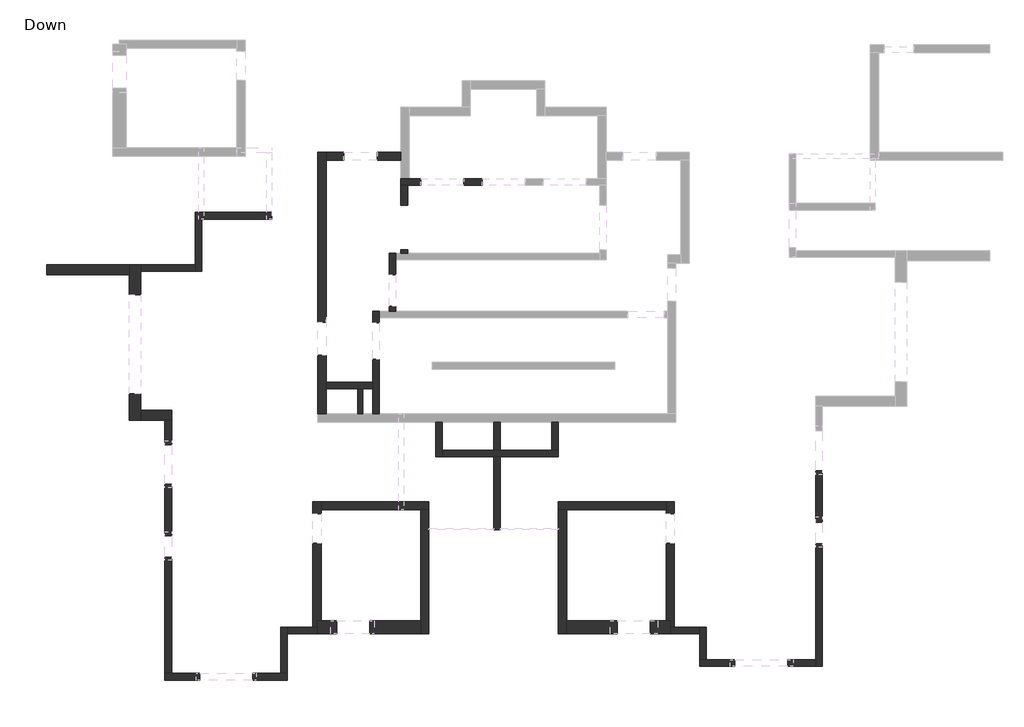
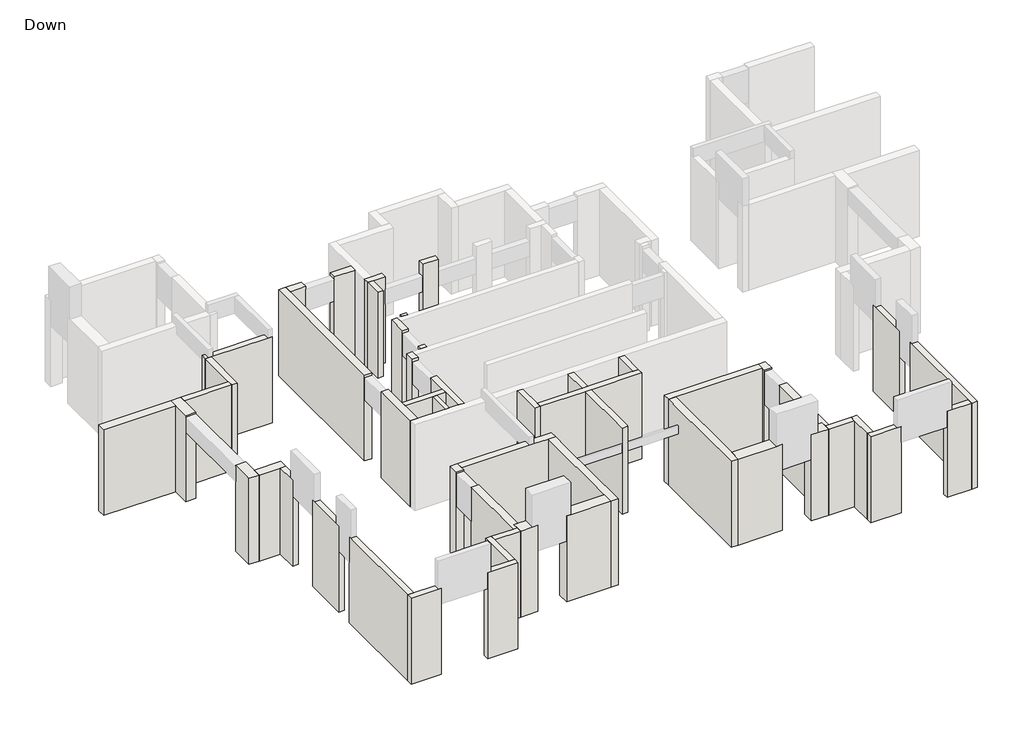
# One storey, part 1 of 3: 51 walls.
# Revit data of these elements (continued)
# Element 19 (IfcWall, "20") (continued)
#   Base Constraint = Down
#   Top Constraint = Typical Floor
#   Materials on its faces: "Concrete"
# Element 20 (IfcWall, "20")
#   Comments = ""
#   Mark = "W54"
#   SOFiSTiK_EdgeZones = "W54"
#   SOFiSTiK_AMG_Comments = ""
#   Top Offset = 0 cm
#   Base Offset = 0 cm
#   wall height = 315 cm
#   SOFiSTiK_AMG_Scheduled = yes
#   SOFiSTiK_AMG_Adjusted = yes
#   Phase Created = New Construction
#   Base Constraint = Down
#   Top Constraint = Typical Floor
#   Materials on its faces: "Concrete"
# Element 21 (IfcWall, "20")
#   Comments = ""
#   Mark = "W55"
#   SOFiSTiK_EdgeZones = "W55"
#   SOFiSTiK_AMG_Comments = ""
#   Top Offset = 0 cm
#   Base Offset = 0 cm
#   wall height = 315 cm
#   SOFiSTiK_AMG_Scheduled = yes
#   SOFiSTiK_AMG_Adjusted = yes
#   Phase Created = New Construction
#   Base Constraint = Down
#   Top Constraint = Typical Floor
#   Materials on its faces: "Concrete"
# Element 22 (IfcWall, "20")
#   Comments = ""
#   Mark = "W56"
#   SOFiSTiK_EdgeZones = "W56"
#   SOFiSTiK_AMG_Comments = ""
#   Top Offset = 0 cm
#   Base Offset = 0 cm
#   wall height = 315 cm
#   SOFiSTiK_AMG_Scheduled = yes
#   SOFiSTiK_AMG_Adjusted = yes
#   Phase Created = New Construction
#   Base Constraint = Down
#   Top Constraint = Typical Floor
#   Materials on its faces: "Concrete"
# Element 23 (IfcWall, "20")
#   Comments = ""
#   Mark = "W57"
#   SOFiSTiK_EdgeZones = "W57"
#   SOFiSTiK_AMG_Comments = ""
#   Top Offset = 0 cm
#   Base Offset = 0 cm
#   wall height = 315 cm
#   SOFiSTiK_AMG_Scheduled = yes
#   SOFiSTiK_AMG_Adjusted = yes
#   Phase Created = New Construction
#   Base Constraint = Down
#   Top Constraint = Typical Floor
#   Materials on its faces: "Concrete"
# Element 24 (IfcWall, "20")
#   Comments = ""
#   Mark = "W58"
#   SOFiSTiK_EdgeZones = "W58"
#   SOFiSTiK_AMG_Comments = ""
#   Top Offset = 0 cm
#   Base Offset = 0 cm
#   wall height = 315 cm
#   SOFiSTiK_AMG_Scheduled = yes
#   SOFiSTiK_AMG_Adjusted = yes
#   Phase Created = New Construction
#   Base Constraint = Down
#   Top Constraint = Typical Floor
#   Materials on its faces: "Concrete"
# Element 25 (IfcWall, "20")
#   Comments = ""
#   Mark = "W59"
#   SOFiSTiK_EdgeZones = "W59"
#   SOFiSTiK_AMG_Comments = ""
#   Top Offset = 0 cm
#   Base Offset = 0 cm
#   wall height = 315 cm
#   SOFiSTiK_AMG_Scheduled = yes
#   SOFiSTiK_AMG_Adjusted = yes
#   Phase Created = New Construction
#   Base Constraint = Down
#   Top Constraint = Typical Floor
#   Materials on its faces: "Concrete"
# Element 26 (IfcWall, "20")
#   Comments = ""
#   Mark = "W60"
#   SOFiSTiK_EdgeZones = "W60"
#   SOFiSTiK_AMG_Comments = ""
#   Top Offset = 0 cm
#   Base Offset = 0 cm
#   wall height = 315 cm
#   SOFiSTiK_AMG_Scheduled = yes
#   SOFiSTiK_AMG_Adjusted = yes
#   Phase Created = New Construction
#   Base Constraint = Down
#   Top Constraint = Typical Floor
#   Materials on its faces: "Concrete"
# Element 27 (IfcWall, "20")
#   Comments = ""
#   Mark = "W61"
#   SOFiSTiK_EdgeZones = "W61"
#   SOFiSTiK_AMG_Comments = ""
#   Top Offset = 0 cm
#   Base Offset = 0 cm
#   wall height = 315 cm
#   SOFiSTiK_AMG_Scheduled = yes
#   SOFiSTiK_AMG_Adjusted = yes
#   Phase Created = New Construction
#   Base Constraint = Down
#   Top Constraint = Typical Floor
#   Materials on its faces: "Concrete"
# Element 28 (IfcWall, "20")
#   Comments = ""
#   Mark = "W69"
#   SOFiSTiK_EdgeZones = "W69"
#   SOFiSTiK_AMG_Comments = ""
#   Top Offset = 0 cm
#   Base Offset = 0 cm
#   wall height = 315 cm
#   SOFiSTiK_AMG_Scheduled = yes
#   SOFiSTiK_AMG_Adjusted = yes
#   Phase Created = New Construction
#   Base Constraint = Down
#   Top Constraint = Typical Floor
#   Materials on its faces: "Concrete"
# Element 29 (IfcWall, "20")
#   Comments = ""
#   Mark = "W71"
#   SOFiSTiK_EdgeZones = "W71"
#   SOFiSTiK_AMG_Comments = ""
#   Top Offset = 0 cm
#   Base Offset = 0 cm
#   wall height = 315 cm
#   SOFiSTiK_AMG_Scheduled = yes
#   SOFiSTiK_AMG_Adjusted = yes
#   Phase Created = New Construction
#   Base Constraint = Down
#   Top Constraint = Typical Floor
#   Materials on its faces: "Concrete"
# Element 30 (IfcWall, "20")
#   Comments = ""
#   Mark = "W72"
#   SOFiSTiK_EdgeZones = "W72"
#   SOFiSTiK_AMG_Comments = ""
#   Top Offset = 0 cm
#   Base Offset = 0 cm
#   wall height = 315 cm
#   SOFiSTiK_AMG_Scheduled = yes
#   SOFiSTiK_AMG_Adjusted = yes
#   Phase Created = New Construction
#   Base Constraint = Down
#   Top Constraint = Typical Floor
#   Materials on its faces: "Concrete"
# Element 31 (IfcWall, "20")
#   Comments = ""
#   Mark = "W73"
#   SOFiSTiK_EdgeZones = "W73"
#   SOFiSTiK_AMG_Comments = ""
#   Top Offset = 0 cm
#   Base Offset = 0 cm
#   wall height = 315 cm
#   SOFiSTiK_AMG_Scheduled = yes
#   SOFiSTiK_AMG_Adjusted = yes
#   Phase Created = New Construction
#   Base Constraint = Down
#   Top Constraint = Typical Floor
#   Materials on its faces: "Concrete"
# Element 32 (IfcWall, "25")
#   Comments = ""
#   Mark = "W90"
#   SOFiSTiK_EdgeZones = "W90"
#   SOFiSTiK_AMG_Comments = ""
#   Top Offset = 0 cm
#   Base Offset = 0 cm
#   wall height = 315 cm
#   SOFiSTiK_AMG_Scheduled = yes
#   SOFiSTiK_AMG_Adjusted = yes
#   Phase Created = New Construction
#   Base Constraint = Down
#   Top Constraint = Typical Floor
#   Materials on its faces: "Concrete"
# Element 33 (IfcWall, "25")
#   Comments = ""
#   Mark = "W91"
#   SOFiSTiK_EdgeZones = "W91"
#   SOFiSTiK_AMG_Comments = ""
#   Top Offset = 0 cm
#   Base Offset = 0 cm
#   wall height = 315 cm
#   SOFiSTiK_AMG_Scheduled = yes
#   SOFiSTiK_AMG_Adjusted = yes
#   Phase Created = New Construction
#   Base Constraint = Down
#   Top Constraint = Typical Floor
#   Materials on its faces: "Concrete"
# Element 34 (IfcWall, "25")
#   Comments = ""
#   Mark = "W92"
#   SOFiSTiK_EdgeZones = "W92"
#   SOFiSTiK_AMG_Comments = ""
#   Top Offset = 0 cm
#   Base Offset = 0 cm
#   wall height = 315 cm
#   SOFiSTiK_AMG_Scheduled = yes
#   SOFiSTiK_AMG_Adjusted = yes
#   Phase Created = New Construction
#   Base Constraint = Down
#   Top Constraint = Typical Floor
#   Materials on its faces: "Concrete"
# Element 35 (IfcWall, "25")
#   Comments = ""
#   Mark = "W93"
#   SOFiSTiK_EdgeZones = "W93"
#   SOFiSTiK_AMG_Comments = ""
#   Top Offset = 0 cm
#   Base Offset = 0 cm
#   wall height = 315 cm
#   SOFiSTiK_AMG_Scheduled = yes
#   SOFiSTiK_AMG_Adjusted = yes
#   Phase Created = New Construction
#   Base Constraint = Down
#   Top Constraint = Typical Floor
#   Materials on its faces: "Concrete"
# Element 36 (IfcWall, "25")
#   Comments = ""
#   Mark = "W94"
#   SOFiSTiK_EdgeZones = "W94"
#   SOFiSTiK_AMG_Comments = ""
#   Top Offset = 0 cm
#   Base Offset = 0 cm
#   wall height = 315 cm
#   SOFiSTiK_AMG_Scheduled = yes
#   SOFiSTiK_AMG_Adjusted = yes
#   Phase Created = New Construction
#   Base Constraint = Down
#   Top Constraint = Typical Floor
#   Materials on its faces: "Concrete"
# Element 37 (IfcWall, "25")
#   Comments = ""
#   Mark = "W95"
#   SOFiSTiK_EdgeZones = "W95"
#   SOFiSTiK_AMG_Comments = ""
#   Top Offset = 0 cm
#   Base Offset = 0 cm
#   wall height = 315 cm
#   SOFiSTiK_AMG_Scheduled = yes
#   SOFiSTiK_AMG_Adjusted = yes
#   Phase Created = New Construction
#   Base Constraint = Down
#   Top Constraint = Typical Floor
#   Materials on its faces: "Concrete"
# Element 38 (IfcWall, "25")
#   Comments = ""
#   Mark = "W96"
#   SOFiSTiK_EdgeZones = "W96"
#   SOFiSTiK_AMG_Comments = ""
#   Top Offset = 0 cm
#   Base Offset = 0 cm
#   wall height = 315 cm
#   SOFiSTiK_AMG_Scheduled = yes
#   SOFiSTiK_AMG_Adjusted = yes
#   Phase Created = New Construction
#   Base Constraint = Down
#   Top Constraint = Typical Floor
#   Materials on its faces: "Concrete"
# Element 39 (IfcWall, "25")
#   Comments = ""
#   Mark = "W97"
#   SOFiSTiK_EdgeZones = "W97"
#   SOFiSTiK_AMG_Comments = ""
#   Top Offset = 0 cm
#   Base Offset = 0 cm
#   wall height = 315 cm
#   SOFiSTiK_AMG_Scheduled = yes
#   SOFiSTiK_AMG_Adjusted = yes
#   Phase Created = New Construction
#   Base Constraint = Down
#   Top Constraint = Typical Floor
#   Materials on its faces: "Concrete"
# Element 40 (IfcWall, "25")
#   Comments = ""
#   Mark = "W100"
#   SOFiSTiK_EdgeZones = "W100"
#   SOFiSTiK_AMG_Comments = ""
#   Top Offset = 0 cm
#   Base Offset = 0 cm
#   wall height = 315 cm
#   SOFiSTiK_AMG_Scheduled = yes
#   SOFiSTiK_AMG_Adjusted = yes
#   Phase Created = New Construction
#   Base Constraint = Down
#   Top Constraint = Typical Floor
#   Materials on its faces: "Concrete"
# Element 41 (IfcWall, "25")
#   Comments = ""
#   Mark = "W101"
#   SOFiSTiK_EdgeZones = "W101"
#   SOFiSTiK_AMG_Comments = ""
#   Top Offset = 0 cm
#   Base Offset = 0 cm
#   wall height = 315 cm
#   SOFiSTiK_AMG_Scheduled = yes
#   SOFiSTiK_AMG_Adjusted = yes
#   Phase Created = New Construction
#   Base Constraint = Down
#   Top Constraint = Typical Floor
#   Materials on its faces: "Concrete"
# Element 42 (IfcWall, "25")
#   Comments = ""
#   Mark = "W102"
#   SOFiSTiK_EdgeZones = "W102"
#   SOFiSTiK_AMG_Comments = ""
#   Top Offset = 0 cm
#   Base Offset = 0 cm
#   wall height = 315 cm
#   SOFiSTiK_AMG_Scheduled = yes
#   SOFiSTiK_AMG_Adjusted = yes
#   Phase Created = New Construction
#   Base Constraint = Down
#   Top Constraint = Typical Floor
#   Materials on its faces: "Concrete"
# Element 43 (IfcWall, "25")
#   Comments = ""
#   Mark = "W103"
#   SOFiSTiK_EdgeZones = "W103"
#   SOFiSTiK_AMG_Comments = ""
#   Top Offset = 0 cm
#   Base Offset = 0 cm
#   wall height = 315 cm
#   SOFiSTiK_AMG_Scheduled = yes
#   SOFiSTiK_AMG_Adjusted = yes
#   Phase Created = New Construction
#   Base Constraint = Down
#   Top Constraint = Typical Floor
#   Materials on its faces: "Concrete"
# Element 44 (IfcWall, "30")
#   Comments = ""
#   Mark = "W77"
#   SOFiSTiK_EdgeZones = "W77"
#   SOFiSTiK_AMG_Comments = ""
#   Top Offset = 0 cm
#   Base Offset = 0 cm
#   wall height = 315 cm
#   SOFiSTiK_AMG_Scheduled = yes
#   SOFiSTiK_AMG_Adjusted = yes
#   Phase Created = New Construction
#   Base Constraint = Down
#   Top Constraint = Typical Floor
#   Materials on its faces: "Concrete"
# Element 45 (IfcWall, "30")
#   Comments = ""
#   Mark = "W78"
#   SOFiSTiK_EdgeZones = "W78"
#   SOFiSTiK_AMG_Comments = ""
#   Top Offset = 0 cm
#   Base Offset = 0 cm
#   wall height = 315 cm
#   SOFiSTiK_AMG_Scheduled = yes
#   SOFiSTiK_AMG_Adjusted = yes
#   Phase Created = New Construction
#   Base Constraint = Down
#   Top Constraint = Typical Floor
#   Materials on its faces: "Concrete"
# Element 46 (IfcWall, "35")
#   Comments = ""
#   Mark = "W9"
#   SOFiSTiK_EdgeZones = "W9"
#   SOFiSTiK_AMG_Comments = ""
#   Top Offset = 0 cm
#   Base Offset = 0 cm
#   wall height = 315 cm
#   SOFiSTiK_AMG_Scheduled = yes
#   SOFiSTiK_AMG_Adjusted = yes
#   Phase Created = New Construction
#   Base Constraint = Down
#   Top Constraint = Typical Floor
#   Materials on its faces: "Concrete"
# Element 47 (IfcWall, "35")
#   Comments = ""
#   Mark = "W10"
#   SOFiSTiK_EdgeZones = "W10"
#   SOFiSTiK_AMG_Comments = ""
#   Top Offset = 0 cm
#   Base Offset = 0 cm
#   wall height = 315 cm
#   SOFiSTiK_AMG_Scheduled = yes
#   SOFiSTiK_AMG_Adjusted = yes
#   Phase Created = New Construction
#   Base Constraint = Down
#   Top Constraint = Typical Floor
#   Materials on its faces: "Concrete"
# Element 48 (IfcWall, "40")
#   Comments = ""
#   Mark = "W118"
#   SOFiSTiK_EdgeZones = "W118"
#   SOFiSTiK_AMG_Comments = ""
#   Top Offset = 0 cm
#   Base Offset = 0 cm
#   wall height = 315 cm
#   SOFiSTiK_AMG_Scheduled = yes
#   SOFiSTiK_AMG_Adjusted = yes
#   Phase Created = New Construction
#   Base Constraint = Down
#   Top Constraint = Typical Floor
#   Materials on its faces: "Concrete"
# Element 49 (IfcWall, "40")
#   Comments = ""
#   Mark = "W119"
#   SOFiSTiK_EdgeZones = "W119"
#   SOFiSTiK_AMG_Comments = ""
#   Top Offset = 0 cm
#   Base Offset = 0 cm
#   wall height = 315 cm
#   SOFiSTiK_AMG_Scheduled = yes
#   SOFiSTiK_AMG_Adjusted = yes
#   Phase Created = New Construction
#   Base Constraint = Down
#   Top Constraint = Typical Floor
#   Materials on its faces: "Concrete"
# Element 50 (IfcWall, "40")
#   Comments = ""
#   Mark = "W122"
#   SOFiSTiK_EdgeZones = "W122"
#   SOFiSTiK_AMG_Comments = ""
#   Top Offset = 0 cm
#   Base Offset = 0 cm
#   wall height = 315 cm
#   SOFiSTiK_AMG_Scheduled = yes
#   SOFiSTiK_AMG_Adjusted = yes
#   Phase Created = New Construction
#   Base Constraint = Down
#   Top Constraint = Typical Floor
#   Materials on its faces: "Concrete"
# Element 51 (IfcWall, "40")
#   Comments = ""
#   Mark = "W123"
#   SOFiSTiK_EdgeZones = "W123"
#   SOFiSTiK_AMG_Comments = ""
#   Top Offset = 0 cm
#   Base Offset = 0 cm
#   wall height = 315 cm
#   SOFiSTiK_AMG_Scheduled = yes
#   SOFiSTiK_AMG_Adjusted = yes
#   Phase Created = New Construction
#   Base Constraint = Down
#   Top Constraint = Typical Floor
#   Materials on its faces: "Concrete"
# Materials
#   "Concrete": class "Concrete", colour RGB 192 192 192, transparency 0, Keynote = "01000", Description = "Cast-in-place concrete", Cost = 0
